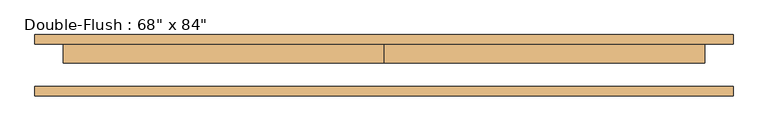
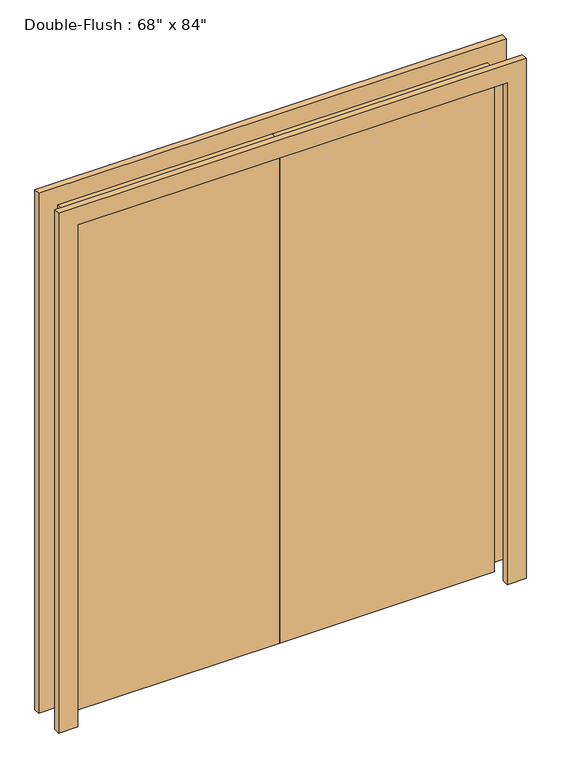
"""IFC4 building model written with IfcOpenShell, lengths in millimetres: door geometry."""

import ifcopenshell
import ifcopenshell.guid

model = None  # the IFC model being written
_history = None  # IfcOwnerHistory: only IFC2X3 demands one
_inside = {}  # id of a spatial element -> (the spatial element, [elements in it])
_under = {}  # id of a project, library or spatial element -> (it, [spatial elements below it])
_declared = {}  # id of a project -> (the project, [libraries it declares])
_typed = {}  # id of a type object -> (the type object, [elements of that type])
_made_of = {}  # id of a material, layer set ... -> (it, [elements and type objects made of it])


def new_model(schema):
    """Start an empty IFC model of exactly this schema.

    Asked for "IFC4X3", IfcOpenShell would pick the latest addendum, in which some entities
    have other attributes; the version numbers below select the first issue.
    IFC2X3 requires an IfcOwnerHistory on every rooted entity: one is made here for all.
    """
    global model, _history
    if schema == "IFC4X3":
        model = ifcopenshell.file(schema_version=(4, 3, 0, 0))
    else:
        model = ifcopenshell.file(schema=schema)
    _inside.clear()
    _under.clear()
    _declared.clear()
    _typed.clear()
    _made_of.clear()
    _history = None
    if model.schema == "IFC2X3":
        org = make("IfcOrganization", Name="unknown")
        user = make(
            "IfcPersonAndOrganization",
            ThePerson=make("IfcPerson", FamilyName="unknown"),
            TheOrganization=org,
        )
        app = make(
            "IfcApplication",
            ApplicationDeveloper=org,
            Version="unknown",
            ApplicationFullName="unknown",
            ApplicationIdentifier="unknown",
        )
        _history = make(
            "IfcOwnerHistory",
            OwningUser=user,
            OwningApplication=app,
            ChangeAction="ADDED",
            CreationDate=0,
        )
    return model


def make(cls, **values):
    """One entity of the class cls with the attributes given. An attribute that is None is left unset."""
    return model.create_entity(
        cls, **{name: value for name, value in values.items() if value is not None}
    )


def rooted(cls, **values):
    """An entity with a GlobalId (a new one), such as an element, a storey or a relation."""
    return make(cls, GlobalId=ifcopenshell.guid.new(), OwnerHistory=_history, **values)


def si_unit(unit_type, name, prefix=None):
    """IfcSIUnit, for example si_unit("LENGTHUNIT", "METRE", prefix="MILLI")."""
    return make("IfcSIUnit", UnitType=unit_type, Prefix=prefix, Name=name)


def assignment(units):
    """IfcUnitAssignment: the units of a project."""
    return None if units is None else make("IfcUnitAssignment", Units=units)


def point(xyz):
    """IfcCartesianPoint."""
    return None if xyz is None else make("IfcCartesianPoint", Coordinates=xyz)


def direction(xyz):
    """IfcDirection."""
    return None if xyz is None else make("IfcDirection", DirectionRatios=xyz)


def frame(location, z_axis=None, x_axis=None):
    """IfcAxis2Placement3D, a coordinate frame: its origin and axes. An axis left out is left unset."""
    return make(
        "IfcAxis2Placement3D",
        Location=point(location),
        Axis=direction(z_axis),
        RefDirection=direction(x_axis),
    )


def origin():
    """The frame at (0, 0, 0) with its axes left unset."""
    return frame((0.0, 0.0, 0.0))


def origin_with_axes():
    """The frame at (0, 0, 0) with the z axis (0, 0, 1) and the x axis (1, 0, 0) written out."""
    return frame((0.0, 0.0, 0.0), z_axis=(0.0, 0.0, 1.0), x_axis=(1.0, 0.0, 0.0))


def place(relative_to, where):
    """IfcLocalPlacement: puts the frame where relative to a parent placement (None: the world)."""
    return make(
        "IfcLocalPlacement", PlacementRelTo=relative_to, RelativePlacement=where
    )


def context(
    kind, dimensions, precision=None, world=None, true_north=None, identifier=None
):
    """IfcGeometricRepresentationContext, for example the 3D "Model" context."""
    return make(
        "IfcGeometricRepresentationContext",
        ContextIdentifier=identifier,
        ContextType=kind,
        CoordinateSpaceDimension=dimensions,
        Precision=precision,
        WorldCoordinateSystem=world,
        TrueNorth=true_north,
    )


def project(units=None, contexts=None):
    """IfcProject with its units and contexts."""
    return rooted(
        "IfcProject",
        Name="project",
        RepresentationContexts=contexts,
        UnitsInContext=assignment(units),
    )


def spatial(cls, under=None, at=None, **own):
    """A site, building, storey or space (cls), placed at a placement, below another one or the project."""
    s = rooted(cls, ObjectPlacement=at, **own)
    if under is not None:
        _under.setdefault(under.id(), (under, []))[1].append(s)
    return s


def polyline(points):
    """IfcPolyline through the points."""
    return make("IfcPolyline", Points=[point(p) for p in points])


def outline(outer, holes=None, kind="AREA"):
    """IfcArbitraryClosedProfileDef: a profile drawn as a closed curve; with holes, ...WithVoids."""
    if holes is None:
        return make("IfcArbitraryClosedProfileDef", ProfileType=kind, OuterCurve=outer)
    return make(
        "IfcArbitraryProfileDefWithVoids",
        ProfileType=kind,
        OuterCurve=outer,
        InnerCurves=holes,
    )


def extrude(swept, where, along, depth):
    """IfcExtrudedAreaSolid: the profile swept, set in the frame where, extruded along a direction by depth."""
    return make(
        "IfcExtrudedAreaSolid",
        SweptArea=swept,
        Position=where,
        ExtrudedDirection=direction(along),
        Depth=depth,
    )


def shape(context_of_items, identifier, shape_type, items):
    """IfcShapeRepresentation: the items that make up one representation, for example the "Body"."""
    return make(
        "IfcShapeRepresentation",
        ContextOfItems=context_of_items,
        RepresentationIdentifier=identifier,
        RepresentationType=shape_type,
        Items=items,
    )


def source(mapping_origin, context_of_items, identifier, shape_type, items):
    """IfcRepresentationMap: a shape defined once, which mapped items show again and again."""
    return make(
        "IfcRepresentationMap",
        MappingOrigin=mapping_origin,
        MappedRepresentation=shape(context_of_items, identifier, shape_type, items),
    )


def transform(
    local_origin,
    x_axis=None,
    y_axis=None,
    z_axis=None,
    scale=None,
    scale2=None,
    scale3=None,
    uniform=True,
):
    """IfcCartesianTransformationOperator3D, or its non-uniform kind. x_axis, y_axis, z_axis: its Axis1, 2, 3."""
    if uniform:
        return make(
            "IfcCartesianTransformationOperator3D",
            Axis1=direction(x_axis),
            Axis2=direction(y_axis),
            LocalOrigin=point(local_origin),
            Scale=scale,
            Axis3=direction(z_axis),
        )
    return make(
        "IfcCartesianTransformationOperator3DnonUniform",
        Axis1=direction(x_axis),
        Axis2=direction(y_axis),
        LocalOrigin=point(local_origin),
        Scale=scale,
        Axis3=direction(z_axis),
        Scale2=scale2,
        Scale3=scale3,
    )


def mapped(mapping_source, mapping_target):
    """IfcMappedItem: shows the shape of a source again, moved by a transform."""
    return make(
        "IfcMappedItem", MappingSource=mapping_source, MappingTarget=mapping_target
    )


def made_of(thing, what):
    """Note that an element or type object is made of a material, layer set ...; save() writes the relation."""
    if what is not None:
        _made_of.setdefault(what.id(), (what, []))[1].append(thing)
    return thing


def element(
    cls,
    number,
    at=None,
    inside=None,
    cuts=None,
    type_object=None,
    material=None,
    context=None,
    identifier="Body",
    shape_type=None,
    held_by="IfcProductDefinitionShape",
    body=None,
    shapes=None,
    **own,
):
    """One element of the class cls, such as IfcWall. Its Tag is "e" and its number.

    at: its placement. inside: the storey or other place that contains it. cuts: it is an
    opening in that element (IfcRelVoidsElement). A single representation is given by context,
    identifier, shape_type and body (its items); several are given by shapes. held_by: the class
    of the entity that holds the representations. save() writes the other relations.
    """
    e = rooted(cls, Tag="e%d" % number, ObjectPlacement=at, **own)
    if body is not None:
        shapes = [shape(context, identifier, shape_type, body)]
    if shapes is not None:
        e.Representation = make(held_by, Representations=shapes)
    if inside is not None:
        _inside.setdefault(inside.id(), (inside, []))[1].append(e)
    if cuts is not None:
        rooted(
            "IfcRelVoidsElement", RelatingBuildingElement=cuts, RelatedOpeningElement=e
        )
    if type_object is not None:
        _typed.setdefault(type_object.id(), (type_object, []))[1].append(e)
    return made_of(e, material)


def aggregate(whole, parts):
    """IfcRelAggregates: a whole, such as a stair, and the parts it consists of."""
    return rooted("IfcRelAggregates", RelatingObject=whole, RelatedObjects=parts)


def save(model, path):
    """Write the relations noted so far, then the file.

    IfcRelAggregates (storeys below a building ...), IfcRelContainedInSpatialStructure (elements
    in a storey), IfcRelDefinesByType, IfcRelAssociatesMaterial and IfcRelDeclares: one each for
    every whole, place, type object, material and project.
    """
    for whole, parts in _under.values():
        aggregate(whole, parts)
    for where, things in _inside.values():
        rooted(
            "IfcRelContainedInSpatialStructure",
            RelatedElements=things,
            RelatingStructure=where,
        )
    for kind, things in _typed.values():
        rooted("IfcRelDefinesByType", RelatedObjects=things, RelatingType=kind)
    for what, things in _made_of.values():
        rooted("IfcRelAssociatesMaterial", RelatedObjects=things, RelatingMaterial=what)
    for by, libraries in _declared.values():
        rooted("IfcRelDeclares", RelatingContext=by, RelatedDefinitions=libraries)
    model.write(path)


def door_80fcf8b2(model_context):
    return source(origin(), model_context, "Body", "SweptSolid", [
        extrude(outline(polyline([(0.0, 57.15), (863.6, 57.15), (863.6, 6.35), (0.0, 6.35), (0.0, 57.15)])), origin_with_axes(), (0.0, 0.0, 1.0), 2133.6),
        extrude(outline(polyline([(-863.6, 57.15), (0.0, 57.15), (0.0, 6.35), (-863.6, 6.35), (-863.6, 57.15)])), origin_with_axes(), (0.0, 0.0, 1.0), 2133.6),
        extrude(outline(polyline([(2133.6, -863.6), (2133.6, 863.6), (0.0, 863.6), (0.0, 939.8), (2209.8, 939.8), (2209.8, -939.8), (0.0, -939.8), (0.0, -863.6), (2133.6, -863.6)])), frame((0.0, -82.55, 0.0), z_axis=(0.0, 1.0, 0.0), x_axis=(0.0, 0.0, 1.0)), (0.0, 0.0, 1.0), 25.4),
        extrude(outline(polyline([(2133.6, -863.6), (2133.6, 863.6), (0.0, 863.6), (0.0, 939.8), (2209.8, 939.8), (2209.8, -939.8), (0.0, -939.8), (0.0, -863.6), (2133.6, -863.6)])), frame((0.0, 57.15, 0.0), z_axis=(0.0, 1.0, 0.0), x_axis=(0.0, 0.0, 1.0)), (0.0, 0.0, 1.0), 25.4),
    ])


if __name__ == "__main__":
    model = new_model("IFC4")
    model_context = context("Model", 3, world=origin())
    ifc_project = project(units=[si_unit("LENGTHUNIT", "METRE", prefix="MILLI")], contexts=[model_context])
    site = spatial("IfcSite", under=ifc_project)
    building = spatial("IfcBuilding", under=site)
    placement = place(None, origin())
    door_shape = door_80fcf8b2(model_context)
    element("IfcDoor", 1, ObjectType="Double-Flush : 68\" x 84\"", at=placement, inside=building, context=model_context, shape_type="MappedRepresentation", body=[
        mapped(door_shape, transform((0.0, 0.0, 0.0), x_axis=(1.0, 0.0, 0.0), y_axis=(0.0, 1.0, 0.0), z_axis=(0.0, 0.0, 1.0))),
    ])
    save(model, "model.ifc")

# Revit data of these elements
# Type "Double-Flush : 68\" x 84\""
#   Type Mark = "10"
#   Assembly Code = "C1020"
#   Thickness = 0' - 2"
#   Height = 7' - 0"
#   Trim Projection Ext = 0' - 1"
#   Trim Projection Int = 0' - 1"
#   Trim Width = 0' - 3"
#   Width = 5' - 8"
#   Function = 0
#   Door Material = Door - Panel
#   Frame Material = Door - Frame
#   Wall Closure = (empty or 0)
# Element 1 (IfcDoor, "Double-Flush : 68\" x 84\"")
#   Materials on its faces: "Door - Frame", "Door - Panel"
# Materials
#   "Door - Panel": class "Wood", colour RGB 230 193 158, transparency 0, Cost = 0
#   "Door - Frame": class "Paint", colour RGB 113 0 0, transparency 0, Cost = 0
